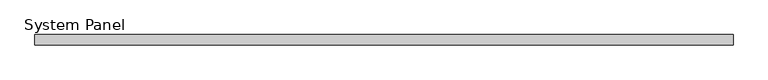
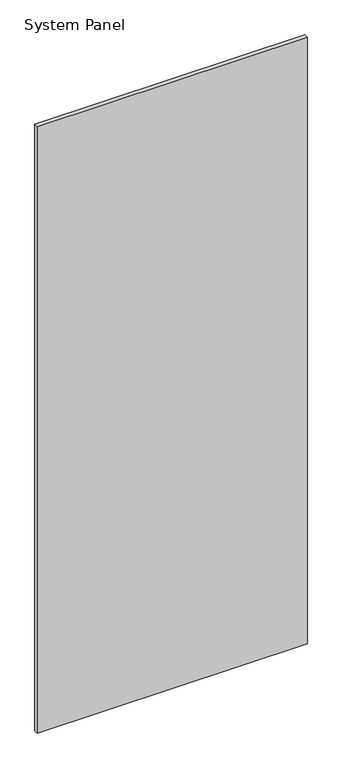
"""IFC4 building model written with IfcOpenShell, lengths in millimetres: plate geometry, System Panel : WWm-Glass-20mm-10mmOffset."""

from ifc_helpers import new_model, si_unit, origin, origin_with_axes, place, context, project, spatial, polyline, outline, extrude, source, transform, mapped, element, save


def system_panel_ff1b972d(model_context):
    return source(origin(), model_context, "Body", "SweptSolid", [
        extrude(outline(polyline([(685.3305698, 0.0), (-685.3305698, 0.0), (-685.3305698, 20.0), (685.3305698, 20.0), (685.3305698, 0.0)])), origin_with_axes(), (0.0, 0.0, 1.0), 3250.0),
    ])


if __name__ == "__main__":
    model = new_model("IFC4")
    model_context = context("Model", 3, world=origin())
    ifc_project = project(units=[si_unit("LENGTHUNIT", "METRE", prefix="MILLI")], contexts=[model_context])
    site = spatial("IfcSite", under=ifc_project)
    building = spatial("IfcBuilding", under=site)
    placement = place(None, origin())
    system_panel_shape = system_panel_ff1b972d(model_context)
    element("IfcPlate", 1, ObjectType="System Panel : WWm-Glass-20mm-10mmOffset", at=placement, inside=building, context=model_context, shape_type="MappedRepresentation", body=[
        mapped(system_panel_shape, transform((0.0, 0.0, 0.0), x_axis=(1.0, 0.0, 0.0), y_axis=(0.0, 1.0, 0.0), z_axis=(0.0, 0.0, 1.0))),
    ])
    save(model, "model.ifc")

# Revit data of these elements
# Type "System Panel : WWm-Glass-20mm-10mmOffset"
#   Finish = ""
# Element 1 (IfcPlate, "System Panel : WWm-Glass-20mm-10mmOffset")
#   Materials on its faces: "WW-EC-GL-Storefront"
# Materials
#   "WW-EC-GL-Storefront": class "Glass", colour RGB 236 240 239, transparency 0.85, Description = "Storefront Glass", Cost = 0
